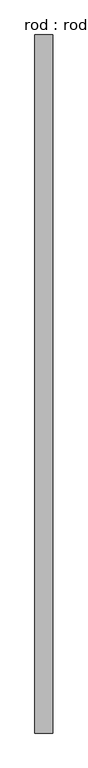
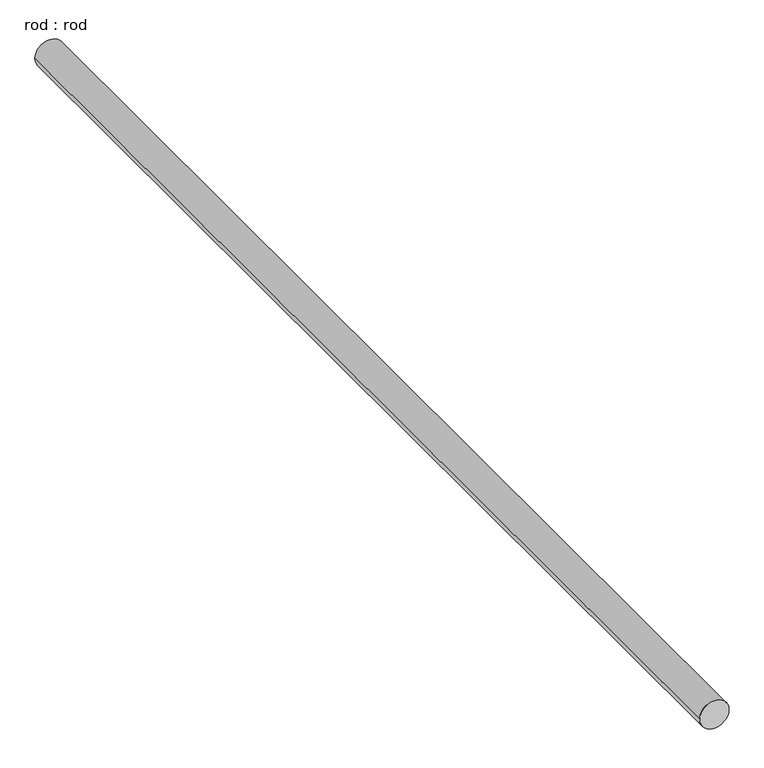
"""IFC4 building model written with IfcOpenShell, lengths in millimetres: proxy geometry, rod : rod."""

from ifc_helpers import new_model, si_unit, point, frame, frame_2d, origin, place, context, project, spatial, circle_curve, trimmed, segment, composite_curve, outline, extrude, source, transform, mapped, element, save


def rod_rod_410e8322(model_context):
    return source(origin(), model_context, "Body", "SweptSolid", [
        extrude(outline(composite_curve([segment(trimmed(circle_curve(frame_2d((0.0108462, 0.0)), 200.0), [point((0.0108462, 200.0))], [point((0.0108462, -200.0))], False, "CARTESIAN"), True, "CONTINUOUS"), segment(trimmed(circle_curve(frame_2d((0.0108462, 0.0)), 200.0), [point((0.0108462, -200.0))], [point((0.0108462, 200.0))], False, "CARTESIAN"), True, "CONTINUOUS")], self_intersect=False)), frame((0.0, -3782.2713847, 0.0), z_axis=(0.0, 1.0, 0.0), x_axis=(0.0, 0.0, 1.0)), (0.0, 0.0, 1.0), 15750.0),
    ])


if __name__ == "__main__":
    model = new_model("IFC4")
    model_context = context("Model", 3, world=origin())
    ifc_project = project(units=[si_unit("LENGTHUNIT", "METRE", prefix="MILLI")], contexts=[model_context])
    site = spatial("IfcSite", under=ifc_project)
    building = spatial("IfcBuilding", under=site)
    placement = place(None, origin())
    rod_rod_shape = rod_rod_410e8322(model_context)
    element("IfcBuildingElementProxy", 1, Name="rod : rod", ObjectType="rod : rod", at=placement, inside=building, context=model_context, shape_type="MappedRepresentation", body=[
        mapped(rod_rod_shape, transform((0.0, 0.0, 0.0), x_axis=(1.0, 0.0, 0.0), y_axis=(0.0, 1.0, 0.0), z_axis=(0.0, 0.0, 1.0))),
    ])
    save(model, "model.ifc")

# Revit data of these elements
# Type "rod : rod"
#   Default Elevation = 0
